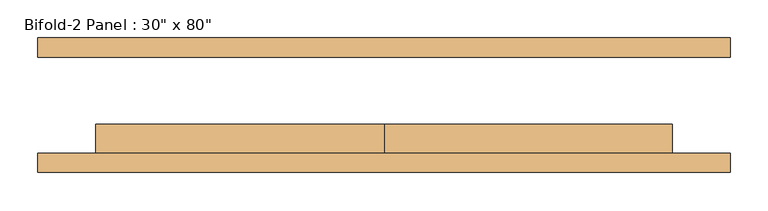
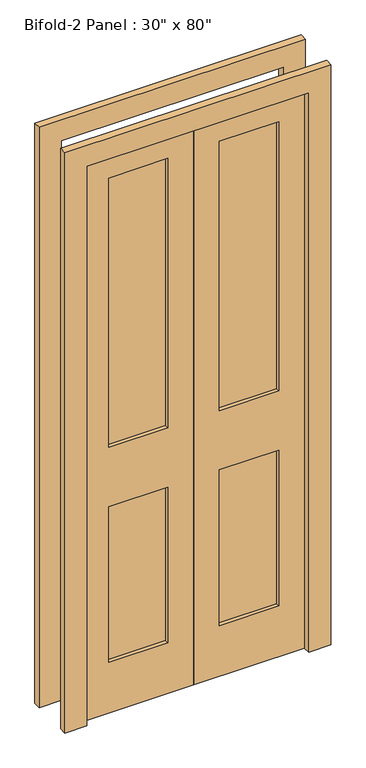
"""IFC4 building model written with IfcOpenShell, lengths in millimetres: door geometry."""

from ifc_helpers import new_model, si_unit, frame, origin, place, context, project, spatial, polyline, outline, extrude, source, transform, mapped, element, save


def door_22ba5e7f(model_context):
    return source(origin(), model_context, "Body", "SweptSolid", [
        extrude(outline(polyline([(2032.0, 0.0), (2032.0, -381.0), (0.0, -381.0), (0.0, 0.0), (2032.0, 0.0)]), holes=[polyline([(1943.1, -88.9), (965.11872, -88.9), (965.11872, -292.1), (1943.1, -292.1), (1943.1, -88.9)]), polyline([(749.3, -88.9), (184.15, -88.9), (184.15, -292.1), (749.3, -292.1), (749.3, -88.9)])]), frame((0.0, -63.5, 0.0), z_axis=(0.0, 1.0, 0.0), x_axis=(0.0, 0.0, 1.0)), (0.0, 0.0, 1.0), 38.1),
        extrude(outline(polyline([(-88.9, -38.1), (-88.9, -50.8), (-292.1, -50.8), (-292.1, -38.1), (-88.9, -38.1)])), frame((0.0, 0.0, 965.11872), z_axis=(0.0, 0.0, 1.0), x_axis=(1.0, 0.0, 0.0)), (0.0, 0.0, 1.0), 977.98128),
        extrude(outline(polyline([(-88.9, -38.1), (-88.9, -50.8), (-292.1, -50.8), (-292.1, -38.1), (-88.9, -38.1)])), frame((0.0, 0.0, 184.15), z_axis=(0.0, 0.0, 1.0), x_axis=(1.0, 0.0, 0.0)), (0.0, 0.0, 1.0), 565.15),
        extrude(outline(polyline([(292.1, -38.1), (292.1, -50.8), (88.9, -50.8), (88.9, -38.1), (292.1, -38.1)])), frame((0.0, 0.0, 965.11872), z_axis=(0.0, 0.0, 1.0), x_axis=(1.0, 0.0, 0.0)), (0.0, 0.0, 1.0), 977.98128),
        extrude(outline(polyline([(292.1, -38.1), (292.1, -50.8), (88.9, -50.8), (88.9, -38.1), (292.1, -38.1)])), frame((0.0, 0.0, 184.15), z_axis=(0.0, 0.0, 1.0), x_axis=(1.0, 0.0, 0.0)), (0.0, 0.0, 1.0), 565.15),
        extrude(outline(polyline([(2108.2, -457.2), (0.0, -457.2), (0.0, -381.0), (2032.0, -381.0), (2032.0, 381.0), (0.0, 381.0), (0.0, 457.2), (2108.2, 457.2), (2108.2, -457.2)])), frame((0.0, -88.9, 0.0), z_axis=(0.0, 1.0, 0.0), x_axis=(0.0, 0.0, 1.0)), (0.0, 0.0, 1.0), 25.4),
        extrude(outline(polyline([(2108.2, 457.2), (2108.2, -457.2), (0.0, -457.2), (0.0, -381.0), (2032.0, -381.0), (2032.0, 381.0), (0.0, 381.0), (0.0, 457.2), (2108.2, 457.2)])), frame((0.0, 63.5, 0.0), z_axis=(0.0, 1.0, 0.0), x_axis=(0.0, 0.0, 1.0)), (0.0, 0.0, 1.0), 25.4),
        extrude(outline(polyline([(2032.0, 381.0), (2032.0, 0.0), (0.0, 0.0), (0.0, 381.0), (2032.0, 381.0)]), holes=[polyline([(1943.1, 88.9), (1943.1, 292.1), (965.11872, 292.1), (965.11872, 88.9), (1943.1, 88.9)]), polyline([(749.3, 88.9), (749.3, 292.1), (184.15, 292.1), (184.15, 88.9), (749.3, 88.9)])]), frame((0.0, -63.5, 0.0), z_axis=(0.0, 1.0, 0.0), x_axis=(0.0, 0.0, 1.0)), (0.0, 0.0, 1.0), 38.1),
    ])


if __name__ == "__main__":
    model = new_model("IFC4")
    model_context = context("Model", 3, world=origin())
    ifc_project = project(units=[si_unit("LENGTHUNIT", "METRE", prefix="MILLI")], contexts=[model_context])
    site = spatial("IfcSite", under=ifc_project)
    building = spatial("IfcBuilding", under=site)
    placement = place(None, origin())
    door_shape = door_22ba5e7f(model_context)
    element("IfcDoor", 1, ObjectType="Bifold-2 Panel : 30\" x 80\"", at=placement, inside=building, context=model_context, shape_type="MappedRepresentation", body=[
        mapped(door_shape, transform((0.0, 0.0, 0.0), x_axis=(1.0, 0.0, 0.0), y_axis=(0.0, 1.0, 0.0), z_axis=(0.0, 0.0, 1.0))),
    ])
    save(model, "model.ifc")

# Revit data of these elements
# Type "Bifold-2 Panel : 30\" x 80\""
#   Type Mark = "11"
#   Construction Type Id = "MDOOR"
#   Assembly Code = "C1020"
#   Analytic Construction = "Metal"
#   Thickness = 0' - 1 1/2"
#   Thermal Resistance (R) = 1.5338 (h·ft²·°F)/BTU
#   Heat Transfer Coefficient (U) = 0.651978 BTU/(h·ft²·°F)
#   Height = 6' - 8"
#   Trim Projection Ext = 0' - 1"
#   Trim Projection Int = 0' - 1"
#   Trim Width = 0' - 3"
#   Width = 2' - 6"
#   Define Thermal Properties by = 1
#   Door Material = Door - Panel
#   Frame Material = Door - Frame
#   Visual Light Transmittance = 0
#   Solar Heat Gain Coefficient = 0
#   Function = (empty or 0)
#   Wall Closure = (empty or 0)
# Element 1 (IfcDoor, "Bifold-2 Panel : 30\" x 80\"")
#   Materials on its faces: "Door - Panel", "Door - Frame"
# Materials
#   "Door - Panel": class "Wood", colour RGB 210 159 95, transparency 0, Cost = 0
#   "Door - Frame": class "Miscellaneous", colour RGB 118 70 51, transparency 0, Cost = 0
